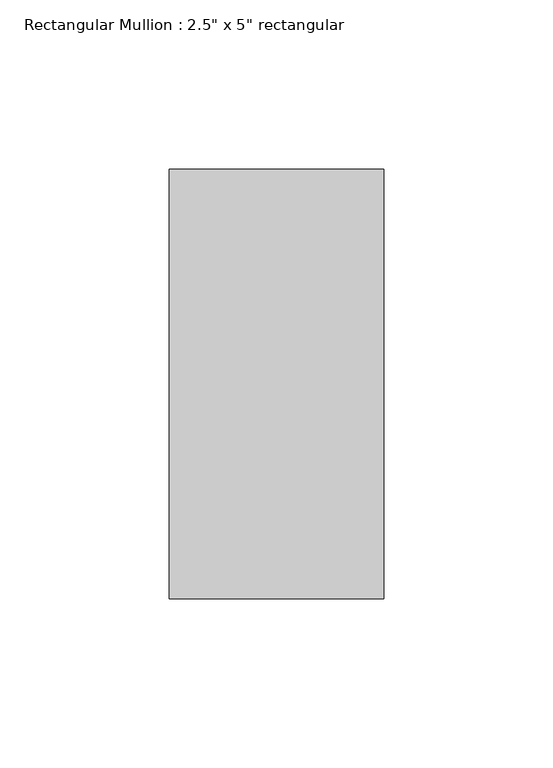
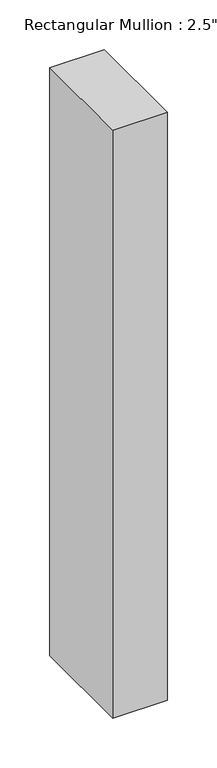
"""IFC4 building model written with IfcOpenShell, lengths in millimetres: member geometry."""

import ifcopenshell
import ifcopenshell.guid

model = None  # the IFC model being written
_history = None  # IfcOwnerHistory: only IFC2X3 demands one
_inside = {}  # id of a spatial element -> (the spatial element, [elements in it])
_under = {}  # id of a project, library or spatial element -> (it, [spatial elements below it])
_declared = {}  # id of a project -> (the project, [libraries it declares])
_typed = {}  # id of a type object -> (the type object, [elements of that type])
_made_of = {}  # id of a material, layer set ... -> (it, [elements and type objects made of it])


def new_model(schema):
    """Start an empty IFC model of exactly this schema.

    Asked for "IFC4X3", IfcOpenShell would pick the latest addendum, in which some entities
    have other attributes; the version numbers below select the first issue.
    IFC2X3 requires an IfcOwnerHistory on every rooted entity: one is made here for all.
    """
    global model, _history
    if schema == "IFC4X3":
        model = ifcopenshell.file(schema_version=(4, 3, 0, 0))
    else:
        model = ifcopenshell.file(schema=schema)
    _inside.clear()
    _under.clear()
    _declared.clear()
    _typed.clear()
    _made_of.clear()
    _history = None
    if model.schema == "IFC2X3":
        org = make("IfcOrganization", Name="unknown")
        user = make(
            "IfcPersonAndOrganization",
            ThePerson=make("IfcPerson", FamilyName="unknown"),
            TheOrganization=org,
        )
        app = make(
            "IfcApplication",
            ApplicationDeveloper=org,
            Version="unknown",
            ApplicationFullName="unknown",
            ApplicationIdentifier="unknown",
        )
        _history = make(
            "IfcOwnerHistory",
            OwningUser=user,
            OwningApplication=app,
            ChangeAction="ADDED",
            CreationDate=0,
        )
    return model


def make(cls, **values):
    """One entity of the class cls with the attributes given. An attribute that is None is left unset."""
    return model.create_entity(
        cls, **{name: value for name, value in values.items() if value is not None}
    )


def rooted(cls, **values):
    """An entity with a GlobalId (a new one), such as an element, a storey or a relation."""
    return make(cls, GlobalId=ifcopenshell.guid.new(), OwnerHistory=_history, **values)


def si_unit(unit_type, name, prefix=None):
    """IfcSIUnit, for example si_unit("LENGTHUNIT", "METRE", prefix="MILLI")."""
    return make("IfcSIUnit", UnitType=unit_type, Prefix=prefix, Name=name)


def assignment(units):
    """IfcUnitAssignment: the units of a project."""
    return None if units is None else make("IfcUnitAssignment", Units=units)


def point(xyz):
    """IfcCartesianPoint."""
    return None if xyz is None else make("IfcCartesianPoint", Coordinates=xyz)


def direction(xyz):
    """IfcDirection."""
    return None if xyz is None else make("IfcDirection", DirectionRatios=xyz)


def frame(location, z_axis=None, x_axis=None):
    """IfcAxis2Placement3D, a coordinate frame: its origin and axes. An axis left out is left unset."""
    return make(
        "IfcAxis2Placement3D",
        Location=point(location),
        Axis=direction(z_axis),
        RefDirection=direction(x_axis),
    )


def origin():
    """The frame at (0, 0, 0) with its axes left unset."""
    return frame((0.0, 0.0, 0.0))


def place(relative_to, where):
    """IfcLocalPlacement: puts the frame where relative to a parent placement (None: the world)."""
    return make(
        "IfcLocalPlacement", PlacementRelTo=relative_to, RelativePlacement=where
    )


def context(
    kind, dimensions, precision=None, world=None, true_north=None, identifier=None
):
    """IfcGeometricRepresentationContext, for example the 3D "Model" context."""
    return make(
        "IfcGeometricRepresentationContext",
        ContextIdentifier=identifier,
        ContextType=kind,
        CoordinateSpaceDimension=dimensions,
        Precision=precision,
        WorldCoordinateSystem=world,
        TrueNorth=true_north,
    )


def project(units=None, contexts=None):
    """IfcProject with its units and contexts."""
    return rooted(
        "IfcProject",
        Name="project",
        RepresentationContexts=contexts,
        UnitsInContext=assignment(units),
    )


def spatial(cls, under=None, at=None, **own):
    """A site, building, storey or space (cls), placed at a placement, below another one or the project."""
    s = rooted(cls, ObjectPlacement=at, **own)
    if under is not None:
        _under.setdefault(under.id(), (under, []))[1].append(s)
    return s


def polyline(points):
    """IfcPolyline through the points."""
    return make("IfcPolyline", Points=[point(p) for p in points])


def outline(outer, holes=None, kind="AREA"):
    """IfcArbitraryClosedProfileDef: a profile drawn as a closed curve; with holes, ...WithVoids."""
    if holes is None:
        return make("IfcArbitraryClosedProfileDef", ProfileType=kind, OuterCurve=outer)
    return make(
        "IfcArbitraryProfileDefWithVoids",
        ProfileType=kind,
        OuterCurve=outer,
        InnerCurves=holes,
    )


def extrude(swept, where, along, depth):
    """IfcExtrudedAreaSolid: the profile swept, set in the frame where, extruded along a direction by depth."""
    return make(
        "IfcExtrudedAreaSolid",
        SweptArea=swept,
        Position=where,
        ExtrudedDirection=direction(along),
        Depth=depth,
    )


def shape(context_of_items, identifier, shape_type, items):
    """IfcShapeRepresentation: the items that make up one representation, for example the "Body"."""
    return make(
        "IfcShapeRepresentation",
        ContextOfItems=context_of_items,
        RepresentationIdentifier=identifier,
        RepresentationType=shape_type,
        Items=items,
    )


def source(mapping_origin, context_of_items, identifier, shape_type, items):
    """IfcRepresentationMap: a shape defined once, which mapped items show again and again."""
    return make(
        "IfcRepresentationMap",
        MappingOrigin=mapping_origin,
        MappedRepresentation=shape(context_of_items, identifier, shape_type, items),
    )


def transform(
    local_origin,
    x_axis=None,
    y_axis=None,
    z_axis=None,
    scale=None,
    scale2=None,
    scale3=None,
    uniform=True,
):
    """IfcCartesianTransformationOperator3D, or its non-uniform kind. x_axis, y_axis, z_axis: its Axis1, 2, 3."""
    if uniform:
        return make(
            "IfcCartesianTransformationOperator3D",
            Axis1=direction(x_axis),
            Axis2=direction(y_axis),
            LocalOrigin=point(local_origin),
            Scale=scale,
            Axis3=direction(z_axis),
        )
    return make(
        "IfcCartesianTransformationOperator3DnonUniform",
        Axis1=direction(x_axis),
        Axis2=direction(y_axis),
        LocalOrigin=point(local_origin),
        Scale=scale,
        Axis3=direction(z_axis),
        Scale2=scale2,
        Scale3=scale3,
    )


def mapped(mapping_source, mapping_target):
    """IfcMappedItem: shows the shape of a source again, moved by a transform."""
    return make(
        "IfcMappedItem", MappingSource=mapping_source, MappingTarget=mapping_target
    )


def made_of(thing, what):
    """Note that an element or type object is made of a material, layer set ...; save() writes the relation."""
    if what is not None:
        _made_of.setdefault(what.id(), (what, []))[1].append(thing)
    return thing


def element(
    cls,
    number,
    at=None,
    inside=None,
    cuts=None,
    type_object=None,
    material=None,
    context=None,
    identifier="Body",
    shape_type=None,
    held_by="IfcProductDefinitionShape",
    body=None,
    shapes=None,
    **own,
):
    """One element of the class cls, such as IfcWall. Its Tag is "e" and its number.

    at: its placement. inside: the storey or other place that contains it. cuts: it is an
    opening in that element (IfcRelVoidsElement). A single representation is given by context,
    identifier, shape_type and body (its items); several are given by shapes. held_by: the class
    of the entity that holds the representations. save() writes the other relations.
    """
    e = rooted(cls, Tag="e%d" % number, ObjectPlacement=at, **own)
    if body is not None:
        shapes = [shape(context, identifier, shape_type, body)]
    if shapes is not None:
        e.Representation = make(held_by, Representations=shapes)
    if inside is not None:
        _inside.setdefault(inside.id(), (inside, []))[1].append(e)
    if cuts is not None:
        rooted(
            "IfcRelVoidsElement", RelatingBuildingElement=cuts, RelatedOpeningElement=e
        )
    if type_object is not None:
        _typed.setdefault(type_object.id(), (type_object, []))[1].append(e)
    return made_of(e, material)


def aggregate(whole, parts):
    """IfcRelAggregates: a whole, such as a stair, and the parts it consists of."""
    return rooted("IfcRelAggregates", RelatingObject=whole, RelatedObjects=parts)


def save(model, path):
    """Write the relations noted so far, then the file.

    IfcRelAggregates (storeys below a building ...), IfcRelContainedInSpatialStructure (elements
    in a storey), IfcRelDefinesByType, IfcRelAssociatesMaterial and IfcRelDeclares: one each for
    every whole, place, type object, material and project.
    """
    for whole, parts in _under.values():
        aggregate(whole, parts)
    for where, things in _inside.values():
        rooted(
            "IfcRelContainedInSpatialStructure",
            RelatedElements=things,
            RelatingStructure=where,
        )
    for kind, things in _typed.values():
        rooted("IfcRelDefinesByType", RelatedObjects=things, RelatingType=kind)
    for what, things in _made_of.values():
        rooted("IfcRelAssociatesMaterial", RelatedObjects=things, RelatingMaterial=what)
    for by, libraries in _declared.values():
        rooted("IfcRelDeclares", RelatingContext=by, RelatedDefinitions=libraries)
    model.write(path)


def member_a43dcf29(model_context):
    return source(origin(), model_context, "Body", "SweptSolid", [
        extrude(outline(polyline([(31.75, 63.5), (31.75, -63.5), (-31.75, -63.5), (-31.75, 63.5), (31.75, 63.5)])), frame((0.0, 0.0, -723.9), z_axis=(0.0, 0.0, 1.0), x_axis=(1.0, 0.0, 0.0)), (0.0, 0.0, 1.0), 723.9),
    ])


if __name__ == "__main__":
    model = new_model("IFC4")
    model_context = context("Model", 3, world=origin())
    ifc_project = project(units=[si_unit("LENGTHUNIT", "METRE", prefix="MILLI")], contexts=[model_context])
    site = spatial("IfcSite", under=ifc_project)
    building = spatial("IfcBuilding", under=site)
    placement = place(None, origin())
    member_shape = member_a43dcf29(model_context)
    element("IfcMember", 1, ObjectType="Rectangular Mullion : 2.5\" x 5\" rectangular", at=placement, inside=building, context=model_context, shape_type="MappedRepresentation", body=[
        mapped(member_shape, transform((0.0, 0.0, 0.0), x_axis=(1.0, 0.0, 0.0), y_axis=(0.0, 1.0, 0.0), z_axis=(0.0, 0.0, 1.0))),
    ])
    save(model, "model.ifc")

# Revit data of these elements
# Type "Rectangular Mullion : 2.5\" x 5\" rectangular"
#   built-in parameter 1007304 = 0.416667 (stored number, unit not read)
#   built-in parameter 1007301 = 0.104167 (stored number, unit not read)
#   built-in parameter 1007300 = 0.104167 (stored number, unit not read)
# Element 1 (IfcMember, "Rectangular Mullion : 2.5\" x 5\" rectangular")
#   Materials on its faces: "Aluminum"
# Materials
#   "Aluminum": class "Metal", colour RGB 247 247 247, transparency 0, Description = "Aluminum 6061", Cost = 0
